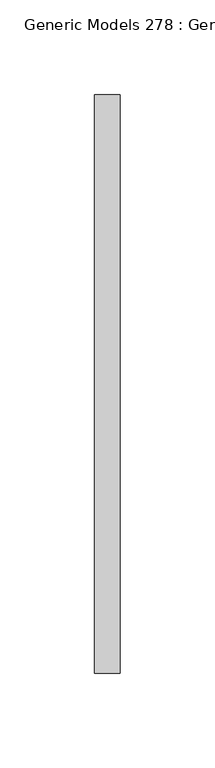
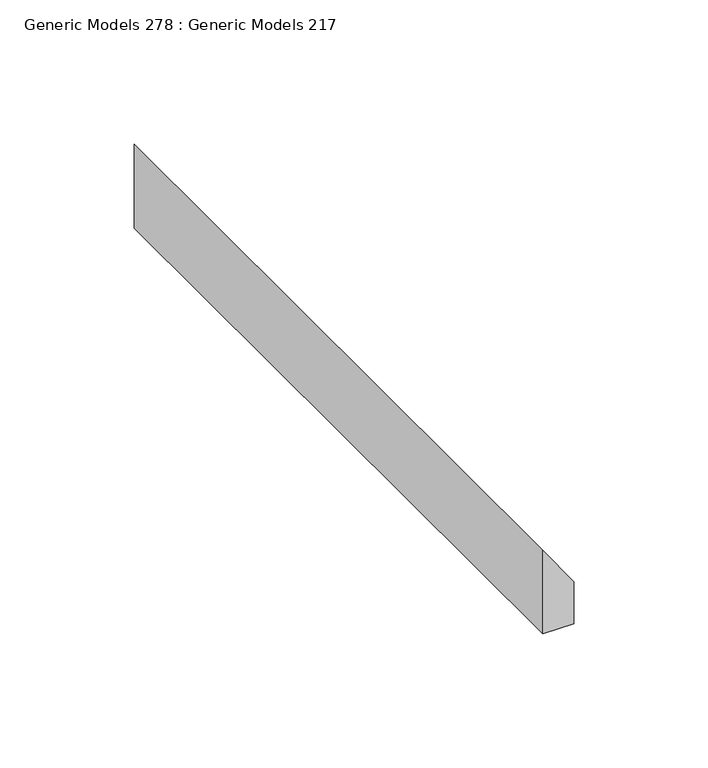
"""IFC4 building model written with IfcOpenShell, lengths in millimetres: proxy geometry, Generic Models 278 : Generic Models 217."""

import ifcopenshell
import ifcopenshell.guid

model = None  # the IFC model being written
_history = None  # IfcOwnerHistory: only IFC2X3 demands one
_inside = {}  # id of a spatial element -> (the spatial element, [elements in it])
_under = {}  # id of a project, library or spatial element -> (it, [spatial elements below it])
_declared = {}  # id of a project -> (the project, [libraries it declares])
_typed = {}  # id of a type object -> (the type object, [elements of that type])
_made_of = {}  # id of a material, layer set ... -> (it, [elements and type objects made of it])


def new_model(schema):
    """Start an empty IFC model of exactly this schema.

    Asked for "IFC4X3", IfcOpenShell would pick the latest addendum, in which some entities
    have other attributes; the version numbers below select the first issue.
    IFC2X3 requires an IfcOwnerHistory on every rooted entity: one is made here for all.
    """
    global model, _history
    if schema == "IFC4X3":
        model = ifcopenshell.file(schema_version=(4, 3, 0, 0))
    else:
        model = ifcopenshell.file(schema=schema)
    _inside.clear()
    _under.clear()
    _declared.clear()
    _typed.clear()
    _made_of.clear()
    _history = None
    if model.schema == "IFC2X3":
        org = make("IfcOrganization", Name="unknown")
        user = make(
            "IfcPersonAndOrganization",
            ThePerson=make("IfcPerson", FamilyName="unknown"),
            TheOrganization=org,
        )
        app = make(
            "IfcApplication",
            ApplicationDeveloper=org,
            Version="unknown",
            ApplicationFullName="unknown",
            ApplicationIdentifier="unknown",
        )
        _history = make(
            "IfcOwnerHistory",
            OwningUser=user,
            OwningApplication=app,
            ChangeAction="ADDED",
            CreationDate=0,
        )
    return model


def make(cls, **values):
    """One entity of the class cls with the attributes given. An attribute that is None is left unset."""
    return model.create_entity(
        cls, **{name: value for name, value in values.items() if value is not None}
    )


def rooted(cls, **values):
    """An entity with a GlobalId (a new one), such as an element, a storey or a relation."""
    return make(cls, GlobalId=ifcopenshell.guid.new(), OwnerHistory=_history, **values)


def si_unit(unit_type, name, prefix=None):
    """IfcSIUnit, for example si_unit("LENGTHUNIT", "METRE", prefix="MILLI")."""
    return make("IfcSIUnit", UnitType=unit_type, Prefix=prefix, Name=name)


def assignment(units):
    """IfcUnitAssignment: the units of a project."""
    return None if units is None else make("IfcUnitAssignment", Units=units)


def point(xyz):
    """IfcCartesianPoint."""
    return None if xyz is None else make("IfcCartesianPoint", Coordinates=xyz)


def direction(xyz):
    """IfcDirection."""
    return None if xyz is None else make("IfcDirection", DirectionRatios=xyz)


def frame(location, z_axis=None, x_axis=None):
    """IfcAxis2Placement3D, a coordinate frame: its origin and axes. An axis left out is left unset."""
    return make(
        "IfcAxis2Placement3D",
        Location=point(location),
        Axis=direction(z_axis),
        RefDirection=direction(x_axis),
    )


def origin():
    """The frame at (0, 0, 0) with its axes left unset."""
    return frame((0.0, 0.0, 0.0))


def place(relative_to, where):
    """IfcLocalPlacement: puts the frame where relative to a parent placement (None: the world)."""
    return make(
        "IfcLocalPlacement", PlacementRelTo=relative_to, RelativePlacement=where
    )


def context(
    kind, dimensions, precision=None, world=None, true_north=None, identifier=None
):
    """IfcGeometricRepresentationContext, for example the 3D "Model" context."""
    return make(
        "IfcGeometricRepresentationContext",
        ContextIdentifier=identifier,
        ContextType=kind,
        CoordinateSpaceDimension=dimensions,
        Precision=precision,
        WorldCoordinateSystem=world,
        TrueNorth=true_north,
    )


def project(units=None, contexts=None):
    """IfcProject with its units and contexts."""
    return rooted(
        "IfcProject",
        Name="project",
        RepresentationContexts=contexts,
        UnitsInContext=assignment(units),
    )


def spatial(cls, under=None, at=None, **own):
    """A site, building, storey or space (cls), placed at a placement, below another one or the project."""
    s = rooted(cls, ObjectPlacement=at, **own)
    if under is not None:
        _under.setdefault(under.id(), (under, []))[1].append(s)
    return s


def polyline(points):
    """IfcPolyline through the points."""
    return make("IfcPolyline", Points=[point(p) for p in points])


def outline(outer, holes=None, kind="AREA"):
    """IfcArbitraryClosedProfileDef: a profile drawn as a closed curve; with holes, ...WithVoids."""
    if holes is None:
        return make("IfcArbitraryClosedProfileDef", ProfileType=kind, OuterCurve=outer)
    return make(
        "IfcArbitraryProfileDefWithVoids",
        ProfileType=kind,
        OuterCurve=outer,
        InnerCurves=holes,
    )


def extrude(swept, where, along, depth):
    """IfcExtrudedAreaSolid: the profile swept, set in the frame where, extruded along a direction by depth."""
    return make(
        "IfcExtrudedAreaSolid",
        SweptArea=swept,
        Position=where,
        ExtrudedDirection=direction(along),
        Depth=depth,
    )


def shape(context_of_items, identifier, shape_type, items):
    """IfcShapeRepresentation: the items that make up one representation, for example the "Body"."""
    return make(
        "IfcShapeRepresentation",
        ContextOfItems=context_of_items,
        RepresentationIdentifier=identifier,
        RepresentationType=shape_type,
        Items=items,
    )


def source(mapping_origin, context_of_items, identifier, shape_type, items):
    """IfcRepresentationMap: a shape defined once, which mapped items show again and again."""
    return make(
        "IfcRepresentationMap",
        MappingOrigin=mapping_origin,
        MappedRepresentation=shape(context_of_items, identifier, shape_type, items),
    )


def transform(
    local_origin,
    x_axis=None,
    y_axis=None,
    z_axis=None,
    scale=None,
    scale2=None,
    scale3=None,
    uniform=True,
):
    """IfcCartesianTransformationOperator3D, or its non-uniform kind. x_axis, y_axis, z_axis: its Axis1, 2, 3."""
    if uniform:
        return make(
            "IfcCartesianTransformationOperator3D",
            Axis1=direction(x_axis),
            Axis2=direction(y_axis),
            LocalOrigin=point(local_origin),
            Scale=scale,
            Axis3=direction(z_axis),
        )
    return make(
        "IfcCartesianTransformationOperator3DnonUniform",
        Axis1=direction(x_axis),
        Axis2=direction(y_axis),
        LocalOrigin=point(local_origin),
        Scale=scale,
        Axis3=direction(z_axis),
        Scale2=scale2,
        Scale3=scale3,
    )


def mapped(mapping_source, mapping_target):
    """IfcMappedItem: shows the shape of a source again, moved by a transform."""
    return make(
        "IfcMappedItem", MappingSource=mapping_source, MappingTarget=mapping_target
    )


def made_of(thing, what):
    """Note that an element or type object is made of a material, layer set ...; save() writes the relation."""
    if what is not None:
        _made_of.setdefault(what.id(), (what, []))[1].append(thing)
    return thing


def element(
    cls,
    number,
    at=None,
    inside=None,
    cuts=None,
    type_object=None,
    material=None,
    context=None,
    identifier="Body",
    shape_type=None,
    held_by="IfcProductDefinitionShape",
    body=None,
    shapes=None,
    **own,
):
    """One element of the class cls, such as IfcWall. Its Tag is "e" and its number.

    at: its placement. inside: the storey or other place that contains it. cuts: it is an
    opening in that element (IfcRelVoidsElement). A single representation is given by context,
    identifier, shape_type and body (its items); several are given by shapes. held_by: the class
    of the entity that holds the representations. save() writes the other relations.
    """
    e = rooted(cls, Tag="e%d" % number, ObjectPlacement=at, **own)
    if body is not None:
        shapes = [shape(context, identifier, shape_type, body)]
    if shapes is not None:
        e.Representation = make(held_by, Representations=shapes)
    if inside is not None:
        _inside.setdefault(inside.id(), (inside, []))[1].append(e)
    if cuts is not None:
        rooted(
            "IfcRelVoidsElement", RelatingBuildingElement=cuts, RelatedOpeningElement=e
        )
    if type_object is not None:
        _typed.setdefault(type_object.id(), (type_object, []))[1].append(e)
    return made_of(e, material)


def aggregate(whole, parts):
    """IfcRelAggregates: a whole, such as a stair, and the parts it consists of."""
    return rooted("IfcRelAggregates", RelatingObject=whole, RelatedObjects=parts)


def save(model, path):
    """Write the relations noted so far, then the file.

    IfcRelAggregates (storeys below a building ...), IfcRelContainedInSpatialStructure (elements
    in a storey), IfcRelDefinesByType, IfcRelAssociatesMaterial and IfcRelDeclares: one each for
    every whole, place, type object, material and project.
    """
    for whole, parts in _under.values():
        aggregate(whole, parts)
    for where, things in _inside.values():
        rooted(
            "IfcRelContainedInSpatialStructure",
            RelatedElements=things,
            RelatingStructure=where,
        )
    for kind, things in _typed.values():
        rooted("IfcRelDefinesByType", RelatedObjects=things, RelatingType=kind)
    for what, things in _made_of.values():
        rooted("IfcRelAssociatesMaterial", RelatedObjects=things, RelatingMaterial=what)
    for by, libraries in _declared.values():
        rooted("IfcRelDeclares", RelatingContext=by, RelatedDefinitions=libraries)
    model.write(path)


def generic_models_278_generic_models_217_487568f1(model_context):
    return source(origin(), model_context, "Body", "SweptSolid", [
        extrude(outline(polyline([(126745.746, 2933.5263704), (126745.746, 2946.9804357), (126764.796, 2946.9804357), (126783.846, 2933.5263704), (126745.746, 2933.5263704)])), frame((0.0, 399.7309662, 0.0), z_axis=(0.0, 1.0, 0.0), x_axis=(0.0, 0.0, 1.0)), (0.0, 0.0, 1.0), 304.8),
    ])


if __name__ == "__main__":
    model = new_model("IFC4")
    model_context = context("Model", 3, world=origin())
    ifc_project = project(units=[si_unit("LENGTHUNIT", "METRE", prefix="MILLI")], contexts=[model_context])
    site = spatial("IfcSite", under=ifc_project)
    building = spatial("IfcBuilding", under=site)
    placement = place(None, origin())
    generic_models_278_generic_models_217_shape = generic_models_278_generic_models_217_487568f1(model_context)
    element("IfcBuildingElementProxy", 1, Name="Generic Models 278 : Generic Models 217", ObjectType="Generic Models 278 : Generic Models 217", at=placement, inside=building, context=model_context, shape_type="MappedRepresentation", body=[
        mapped(generic_models_278_generic_models_217_shape, transform((0.0, 0.0, 0.0), x_axis=(1.0, 0.0, 0.0), y_axis=(0.0, 1.0, 0.0), z_axis=(0.0, 0.0, 1.0))),
    ])
    save(model, "model.ifc")

# Revit data of these elements
# Element 1 (IfcBuildingElementProxy, "Generic Models 278 : Generic Models 217")
#   Materials on its faces: "_WOOD FLOORING (SPEC T.B.D.)"
# Materials
#   "_WOOD FLOORING (SPEC T.B.D.)": class "Generic", colour RGB 177 130 114, transparency 0, Cost = 0
